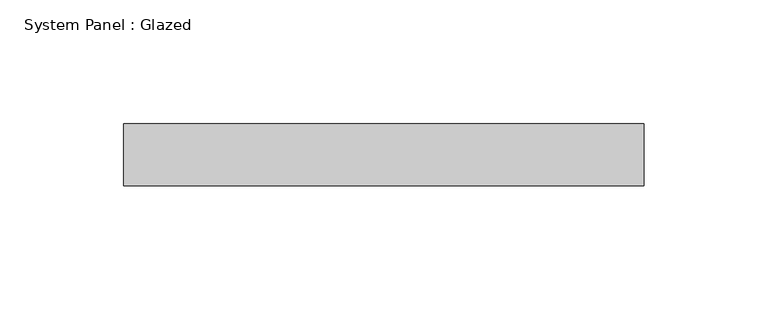
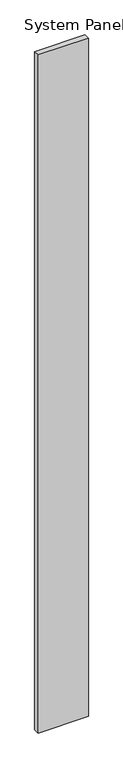
"""IFC4 building model written with IfcOpenShell, lengths in millimetres: plate geometry, System Panel : Glazed."""

from ifc_helpers import new_model, si_unit, origin, origin_with_axes, place, context, project, spatial, polyline, outline, extrude, source, transform, mapped, element, save


def system_panel_glazed_34b19285(model_context):
    return source(origin(), model_context, "Body", "SweptSolid", [
        extrude(outline(polyline([(104.9999998, 24.5), (-104.9999998, 24.5), (-104.9999998, 49.5), (104.9999998, 49.5), (104.9999998, 24.5)])), origin_with_axes(), (0.0, 0.0, 1.0), 3000.0),
    ])


if __name__ == "__main__":
    model = new_model("IFC4")
    model_context = context("Model", 3, world=origin())
    ifc_project = project(units=[si_unit("LENGTHUNIT", "METRE", prefix="MILLI")], contexts=[model_context])
    site = spatial("IfcSite", under=ifc_project)
    building = spatial("IfcBuilding", under=site)
    placement = place(None, origin())
    system_panel_glazed_shape = system_panel_glazed_34b19285(model_context)
    element("IfcPlate", 1, ObjectType="System Panel : Glazed", at=placement, inside=building, context=model_context, shape_type="MappedRepresentation", body=[
        mapped(system_panel_glazed_shape, transform((0.0, 0.0, 0.0), x_axis=(1.0, 0.0, 0.0), y_axis=(0.0, 1.0, 0.0), z_axis=(0.0, 0.0, 1.0))),
    ])
    save(model, "model.ifc")

# Revit data of these elements
# Type "System Panel : Glazed"
#   Construction Type Id = "GSP4R"
#   Analytic Construction = "1/8 in Pilkington single glazing"
#   Visual Light Transmittance = 0.9
#   Solar Heat Gain Coefficient = 0.86
#   Heat Transfer Coefficient (U) = 6.7069 W/(m²·K)
#   Define Thermal Properties by = 1
# Element 1 (IfcPlate, "System Panel : Glazed")
#   Materials on its faces: "Glass"
# Materials
#   "Glass": class "Glass", colour RGB 0 128 192, transparency 0.9, Description = "Soda Lime Glass", Cost = 0
